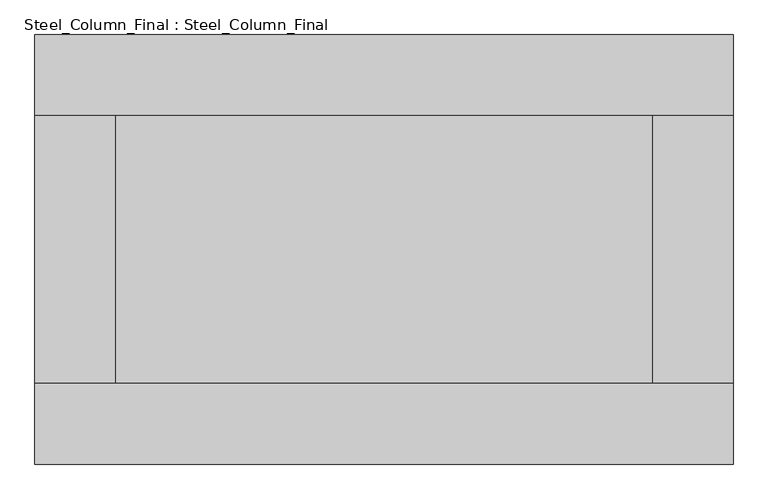
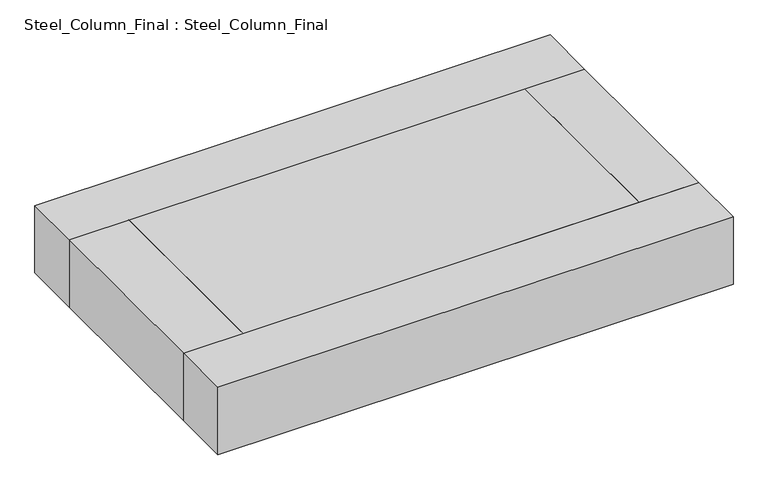
"""IFC4 building model written with IfcOpenShell, lengths in millimetres: proxy geometry, Steel_Column_Final : Steel_Column_Final."""

import ifcopenshell
import ifcopenshell.guid

model = None  # the IFC model being written
_history = None  # IfcOwnerHistory: only IFC2X3 demands one
_inside = {}  # id of a spatial element -> (the spatial element, [elements in it])
_under = {}  # id of a project, library or spatial element -> (it, [spatial elements below it])
_declared = {}  # id of a project -> (the project, [libraries it declares])
_typed = {}  # id of a type object -> (the type object, [elements of that type])
_made_of = {}  # id of a material, layer set ... -> (it, [elements and type objects made of it])


def new_model(schema):
    """Start an empty IFC model of exactly this schema.

    Asked for "IFC4X3", IfcOpenShell would pick the latest addendum, in which some entities
    have other attributes; the version numbers below select the first issue.
    IFC2X3 requires an IfcOwnerHistory on every rooted entity: one is made here for all.
    """
    global model, _history
    if schema == "IFC4X3":
        model = ifcopenshell.file(schema_version=(4, 3, 0, 0))
    else:
        model = ifcopenshell.file(schema=schema)
    _inside.clear()
    _under.clear()
    _declared.clear()
    _typed.clear()
    _made_of.clear()
    _history = None
    if model.schema == "IFC2X3":
        org = make("IfcOrganization", Name="unknown")
        user = make(
            "IfcPersonAndOrganization",
            ThePerson=make("IfcPerson", FamilyName="unknown"),
            TheOrganization=org,
        )
        app = make(
            "IfcApplication",
            ApplicationDeveloper=org,
            Version="unknown",
            ApplicationFullName="unknown",
            ApplicationIdentifier="unknown",
        )
        _history = make(
            "IfcOwnerHistory",
            OwningUser=user,
            OwningApplication=app,
            ChangeAction="ADDED",
            CreationDate=0,
        )
    return model


def make(cls, **values):
    """One entity of the class cls with the attributes given. An attribute that is None is left unset."""
    return model.create_entity(
        cls, **{name: value for name, value in values.items() if value is not None}
    )


def rooted(cls, **values):
    """An entity with a GlobalId (a new one), such as an element, a storey or a relation."""
    return make(cls, GlobalId=ifcopenshell.guid.new(), OwnerHistory=_history, **values)


def si_unit(unit_type, name, prefix=None):
    """IfcSIUnit, for example si_unit("LENGTHUNIT", "METRE", prefix="MILLI")."""
    return make("IfcSIUnit", UnitType=unit_type, Prefix=prefix, Name=name)


def assignment(units):
    """IfcUnitAssignment: the units of a project."""
    return None if units is None else make("IfcUnitAssignment", Units=units)


def point(xyz):
    """IfcCartesianPoint."""
    return None if xyz is None else make("IfcCartesianPoint", Coordinates=xyz)


def direction(xyz):
    """IfcDirection."""
    return None if xyz is None else make("IfcDirection", DirectionRatios=xyz)


def frame(location, z_axis=None, x_axis=None):
    """IfcAxis2Placement3D, a coordinate frame: its origin and axes. An axis left out is left unset."""
    return make(
        "IfcAxis2Placement3D",
        Location=point(location),
        Axis=direction(z_axis),
        RefDirection=direction(x_axis),
    )


def origin():
    """The frame at (0, 0, 0) with its axes left unset."""
    return frame((0.0, 0.0, 0.0))


def place(relative_to, where):
    """IfcLocalPlacement: puts the frame where relative to a parent placement (None: the world)."""
    return make(
        "IfcLocalPlacement", PlacementRelTo=relative_to, RelativePlacement=where
    )


def context(
    kind, dimensions, precision=None, world=None, true_north=None, identifier=None
):
    """IfcGeometricRepresentationContext, for example the 3D "Model" context."""
    return make(
        "IfcGeometricRepresentationContext",
        ContextIdentifier=identifier,
        ContextType=kind,
        CoordinateSpaceDimension=dimensions,
        Precision=precision,
        WorldCoordinateSystem=world,
        TrueNorth=true_north,
    )


def project(units=None, contexts=None):
    """IfcProject with its units and contexts."""
    return rooted(
        "IfcProject",
        Name="project",
        RepresentationContexts=contexts,
        UnitsInContext=assignment(units),
    )


def spatial(cls, under=None, at=None, **own):
    """A site, building, storey or space (cls), placed at a placement, below another one or the project."""
    s = rooted(cls, ObjectPlacement=at, **own)
    if under is not None:
        _under.setdefault(under.id(), (under, []))[1].append(s)
    return s


def polyline(points):
    """IfcPolyline through the points."""
    return make("IfcPolyline", Points=[point(p) for p in points])


def outline(outer, holes=None, kind="AREA"):
    """IfcArbitraryClosedProfileDef: a profile drawn as a closed curve; with holes, ...WithVoids."""
    if holes is None:
        return make("IfcArbitraryClosedProfileDef", ProfileType=kind, OuterCurve=outer)
    return make(
        "IfcArbitraryProfileDefWithVoids",
        ProfileType=kind,
        OuterCurve=outer,
        InnerCurves=holes,
    )


def extrude(swept, where, along, depth):
    """IfcExtrudedAreaSolid: the profile swept, set in the frame where, extruded along a direction by depth."""
    return make(
        "IfcExtrudedAreaSolid",
        SweptArea=swept,
        Position=where,
        ExtrudedDirection=direction(along),
        Depth=depth,
    )


def shape(context_of_items, identifier, shape_type, items):
    """IfcShapeRepresentation: the items that make up one representation, for example the "Body"."""
    return make(
        "IfcShapeRepresentation",
        ContextOfItems=context_of_items,
        RepresentationIdentifier=identifier,
        RepresentationType=shape_type,
        Items=items,
    )


def source(mapping_origin, context_of_items, identifier, shape_type, items):
    """IfcRepresentationMap: a shape defined once, which mapped items show again and again."""
    return make(
        "IfcRepresentationMap",
        MappingOrigin=mapping_origin,
        MappedRepresentation=shape(context_of_items, identifier, shape_type, items),
    )


def transform(
    local_origin,
    x_axis=None,
    y_axis=None,
    z_axis=None,
    scale=None,
    scale2=None,
    scale3=None,
    uniform=True,
):
    """IfcCartesianTransformationOperator3D, or its non-uniform kind. x_axis, y_axis, z_axis: its Axis1, 2, 3."""
    if uniform:
        return make(
            "IfcCartesianTransformationOperator3D",
            Axis1=direction(x_axis),
            Axis2=direction(y_axis),
            LocalOrigin=point(local_origin),
            Scale=scale,
            Axis3=direction(z_axis),
        )
    return make(
        "IfcCartesianTransformationOperator3DnonUniform",
        Axis1=direction(x_axis),
        Axis2=direction(y_axis),
        LocalOrigin=point(local_origin),
        Scale=scale,
        Axis3=direction(z_axis),
        Scale2=scale2,
        Scale3=scale3,
    )


def mapped(mapping_source, mapping_target):
    """IfcMappedItem: shows the shape of a source again, moved by a transform."""
    return make(
        "IfcMappedItem", MappingSource=mapping_source, MappingTarget=mapping_target
    )


def made_of(thing, what):
    """Note that an element or type object is made of a material, layer set ...; save() writes the relation."""
    if what is not None:
        _made_of.setdefault(what.id(), (what, []))[1].append(thing)
    return thing


def element(
    cls,
    number,
    at=None,
    inside=None,
    cuts=None,
    type_object=None,
    material=None,
    context=None,
    identifier="Body",
    shape_type=None,
    held_by="IfcProductDefinitionShape",
    body=None,
    shapes=None,
    **own,
):
    """One element of the class cls, such as IfcWall. Its Tag is "e" and its number.

    at: its placement. inside: the storey or other place that contains it. cuts: it is an
    opening in that element (IfcRelVoidsElement). A single representation is given by context,
    identifier, shape_type and body (its items); several are given by shapes. held_by: the class
    of the entity that holds the representations. save() writes the other relations.
    """
    e = rooted(cls, Tag="e%d" % number, ObjectPlacement=at, **own)
    if body is not None:
        shapes = [shape(context, identifier, shape_type, body)]
    if shapes is not None:
        e.Representation = make(held_by, Representations=shapes)
    if inside is not None:
        _inside.setdefault(inside.id(), (inside, []))[1].append(e)
    if cuts is not None:
        rooted(
            "IfcRelVoidsElement", RelatingBuildingElement=cuts, RelatedOpeningElement=e
        )
    if type_object is not None:
        _typed.setdefault(type_object.id(), (type_object, []))[1].append(e)
    return made_of(e, material)


def aggregate(whole, parts):
    """IfcRelAggregates: a whole, such as a stair, and the parts it consists of."""
    return rooted("IfcRelAggregates", RelatingObject=whole, RelatedObjects=parts)


def save(model, path):
    """Write the relations noted so far, then the file.

    IfcRelAggregates (storeys below a building ...), IfcRelContainedInSpatialStructure (elements
    in a storey), IfcRelDefinesByType, IfcRelAssociatesMaterial and IfcRelDeclares: one each for
    every whole, place, type object, material and project.
    """
    for whole, parts in _under.values():
        aggregate(whole, parts)
    for where, things in _inside.values():
        rooted(
            "IfcRelContainedInSpatialStructure",
            RelatedElements=things,
            RelatingStructure=where,
        )
    for kind, things in _typed.values():
        rooted("IfcRelDefinesByType", RelatedObjects=things, RelatingType=kind)
    for what, things in _made_of.values():
        rooted("IfcRelAssociatesMaterial", RelatedObjects=things, RelatingMaterial=what)
    for by, libraries in _declared.values():
        rooted("IfcRelDeclares", RelatingContext=by, RelatedDefinitions=libraries)
    model.write(path)


def steel_column_final_steel_column_final_81049bd6(model_context):
    return source(origin(), model_context, "Body", "SweptSolid", [
        extrude(outline(polyline([(6500.0, 2500.0), (-6500.0, 2500.0), (-6500.0, 4000.0), (6500.0, 4000.0), (6500.0, 2500.0)])), frame((0.0, 0.0, 130700.0), z_axis=(0.0, 0.0, 1.0), x_axis=(1.0, 0.0, 0.0)), (0.0, 0.0, 1.0), 1800.0),
        extrude(outline(polyline([(-6500.0, -2500.0), (6500.0, -2500.0), (6500.0, -4000.0), (-6500.0, -4000.0), (-6500.0, -2500.0)])), frame((0.0, 0.0, 130700.0), z_axis=(0.0, 0.0, 1.0), x_axis=(1.0, 0.0, 0.0)), (0.0, 0.0, 1.0), 1800.0),
        extrude(outline(polyline([(5000.0, -2500.0), (5000.0, 2500.0), (6500.0, 2500.0), (6500.0, -2500.0), (5000.0, -2500.0)])), frame((0.0, 0.0, 130700.0), z_axis=(0.0, 0.0, 1.0), x_axis=(1.0, 0.0, 0.0)), (0.0, 0.0, 1.0), 1800.0),
        extrude(outline(polyline([(-5000.0, 2500.0), (-5000.0, -2500.0), (-6500.0, -2500.0), (-6500.0, 2500.0), (-5000.0, 2500.0)])), frame((0.0, 0.0, 130700.0), z_axis=(0.0, 0.0, 1.0), x_axis=(1.0, 0.0, 0.0)), (0.0, 0.0, 1.0), 1800.0),
        extrude(outline(polyline([(-5000.0, -2500.0), (-5000.0, 2500.0), (5000.0, 2500.0), (5000.0, -2500.0), (-5000.0, -2500.0)])), frame((0.0, 0.0, 130700.0), z_axis=(0.0, 0.0, 1.0), x_axis=(1.0, 0.0, 0.0)), (0.0, 0.0, 1.0), 1800.0),
    ])


if __name__ == "__main__":
    model = new_model("IFC4")
    model_context = context("Model", 3, world=origin())
    ifc_project = project(units=[si_unit("LENGTHUNIT", "METRE", prefix="MILLI")], contexts=[model_context])
    site = spatial("IfcSite", under=ifc_project)
    building = spatial("IfcBuilding", under=site)
    placement = place(None, origin())
    steel_column_final_steel_column_final_shape = steel_column_final_steel_column_final_81049bd6(model_context)
    element("IfcBuildingElementProxy", 1, Name="Steel_Column_Final : Steel_Column_Final", ObjectType="Steel_Column_Final : Steel_Column_Final", at=placement, inside=building, context=model_context, shape_type="MappedRepresentation", body=[
        mapped(steel_column_final_steel_column_final_shape, transform((0.0, 0.0, 0.0), x_axis=(1.0, 0.0, 0.0), y_axis=(0.0, 1.0, 0.0), z_axis=(0.0, 0.0, 1.0))),
    ])
    save(model, "model.ifc")

# Revit data of these elements
# Type "Steel_Column_Final : Steel_Column_Final"
#   Top Width [instance default] = 5000 mm
#   Top Length = 10000 mm
#   Length = 21000 mm
#   Height [instance default] = 50000 mm
#   Bottom Width [instance default] = 5000 mm
#   Default Elevation = 0
# Element 1 (IfcBuildingElementProxy, "Steel_Column_Final : Steel_Column_Final")
#   Height = 130700 mm
